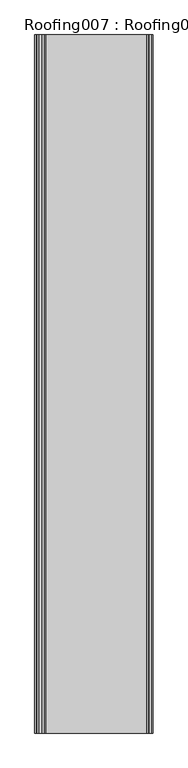
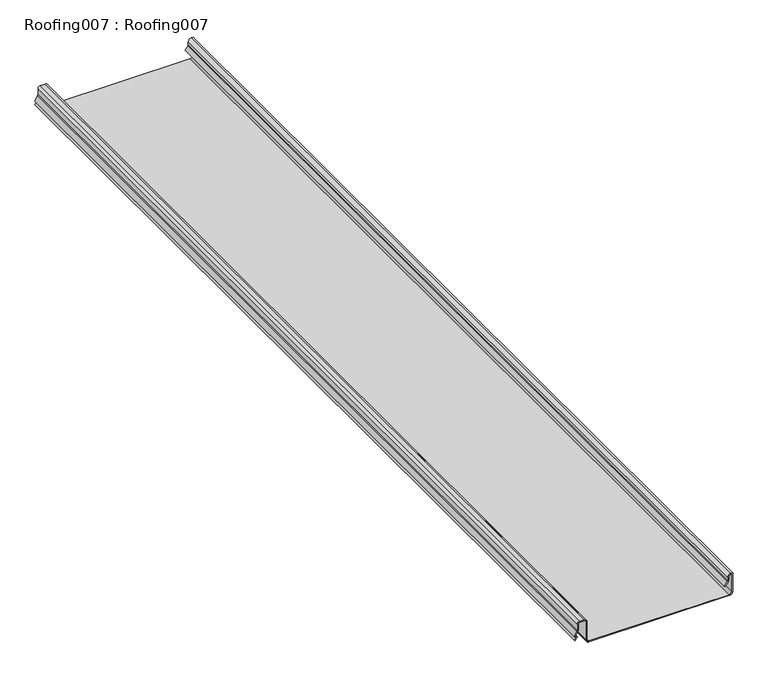
"""IFC4 building model written with IfcOpenShell, lengths in millimetres: proxy geometry, Roofing007 : Roofing007."""

import ifcopenshell
import ifcopenshell.guid

model = None  # the IFC model being written
_history = None  # IfcOwnerHistory: only IFC2X3 demands one
_inside = {}  # id of a spatial element -> (the spatial element, [elements in it])
_under = {}  # id of a project, library or spatial element -> (it, [spatial elements below it])
_declared = {}  # id of a project -> (the project, [libraries it declares])
_typed = {}  # id of a type object -> (the type object, [elements of that type])
_made_of = {}  # id of a material, layer set ... -> (it, [elements and type objects made of it])


def new_model(schema):
    """Start an empty IFC model of exactly this schema.

    Asked for "IFC4X3", IfcOpenShell would pick the latest addendum, in which some entities
    have other attributes; the version numbers below select the first issue.
    IFC2X3 requires an IfcOwnerHistory on every rooted entity: one is made here for all.
    """
    global model, _history
    if schema == "IFC4X3":
        model = ifcopenshell.file(schema_version=(4, 3, 0, 0))
    else:
        model = ifcopenshell.file(schema=schema)
    _inside.clear()
    _under.clear()
    _declared.clear()
    _typed.clear()
    _made_of.clear()
    _history = None
    if model.schema == "IFC2X3":
        org = make("IfcOrganization", Name="unknown")
        user = make(
            "IfcPersonAndOrganization",
            ThePerson=make("IfcPerson", FamilyName="unknown"),
            TheOrganization=org,
        )
        app = make(
            "IfcApplication",
            ApplicationDeveloper=org,
            Version="unknown",
            ApplicationFullName="unknown",
            ApplicationIdentifier="unknown",
        )
        _history = make(
            "IfcOwnerHistory",
            OwningUser=user,
            OwningApplication=app,
            ChangeAction="ADDED",
            CreationDate=0,
        )
    return model


def make(cls, **values):
    """One entity of the class cls with the attributes given. An attribute that is None is left unset."""
    return model.create_entity(
        cls, **{name: value for name, value in values.items() if value is not None}
    )


def rooted(cls, **values):
    """An entity with a GlobalId (a new one), such as an element, a storey or a relation."""
    return make(cls, GlobalId=ifcopenshell.guid.new(), OwnerHistory=_history, **values)


def si_unit(unit_type, name, prefix=None):
    """IfcSIUnit, for example si_unit("LENGTHUNIT", "METRE", prefix="MILLI")."""
    return make("IfcSIUnit", UnitType=unit_type, Prefix=prefix, Name=name)


def assignment(units):
    """IfcUnitAssignment: the units of a project."""
    return None if units is None else make("IfcUnitAssignment", Units=units)


def point(xyz):
    """IfcCartesianPoint."""
    return None if xyz is None else make("IfcCartesianPoint", Coordinates=xyz)


def direction(xyz):
    """IfcDirection."""
    return None if xyz is None else make("IfcDirection", DirectionRatios=xyz)


def frame(location, z_axis=None, x_axis=None):
    """IfcAxis2Placement3D, a coordinate frame: its origin and axes. An axis left out is left unset."""
    return make(
        "IfcAxis2Placement3D",
        Location=point(location),
        Axis=direction(z_axis),
        RefDirection=direction(x_axis),
    )


def frame_2d(location, x_axis=None):
    """IfcAxis2Placement2D, a coordinate frame in the plane: its origin and x axis."""
    return make(
        "IfcAxis2Placement2D", Location=point(location), RefDirection=direction(x_axis)
    )


def origin():
    """The frame at (0, 0, 0) with its axes left unset."""
    return frame((0.0, 0.0, 0.0))


def place(relative_to, where):
    """IfcLocalPlacement: puts the frame where relative to a parent placement (None: the world)."""
    return make(
        "IfcLocalPlacement", PlacementRelTo=relative_to, RelativePlacement=where
    )


def context(
    kind, dimensions, precision=None, world=None, true_north=None, identifier=None
):
    """IfcGeometricRepresentationContext, for example the 3D "Model" context."""
    return make(
        "IfcGeometricRepresentationContext",
        ContextIdentifier=identifier,
        ContextType=kind,
        CoordinateSpaceDimension=dimensions,
        Precision=precision,
        WorldCoordinateSystem=world,
        TrueNorth=true_north,
    )


def project(units=None, contexts=None):
    """IfcProject with its units and contexts."""
    return rooted(
        "IfcProject",
        Name="project",
        RepresentationContexts=contexts,
        UnitsInContext=assignment(units),
    )


def spatial(cls, under=None, at=None, **own):
    """A site, building, storey or space (cls), placed at a placement, below another one or the project."""
    s = rooted(cls, ObjectPlacement=at, **own)
    if under is not None:
        _under.setdefault(under.id(), (under, []))[1].append(s)
    return s


def polyline(points):
    """IfcPolyline through the points."""
    return make("IfcPolyline", Points=[point(p) for p in points])


def circle_curve(where, radius):
    """IfcCircle in the frame where."""
    return make("IfcCircle", Position=where, Radius=radius)


def trimmed(basis, trim1, trim2, sense, master):
    """IfcTrimmedCurve: the piece of a basis curve between two trims."""
    return make(
        "IfcTrimmedCurve",
        BasisCurve=basis,
        Trim1=trim1,
        Trim2=trim2,
        SenseAgreement=sense,
        MasterRepresentation=master,
    )


def segment(curve, same_sense, transition):
    """IfcCompositeCurveSegment."""
    return make(
        "IfcCompositeCurveSegment",
        Transition=transition,
        SameSense=same_sense,
        ParentCurve=curve,
    )


def composite_curve(segments, self_intersect=None):
    """IfcCompositeCurve: segments joined end to end."""
    return make("IfcCompositeCurve", Segments=segments, SelfIntersect=self_intersect)


def outline(outer, holes=None, kind="AREA"):
    """IfcArbitraryClosedProfileDef: a profile drawn as a closed curve; with holes, ...WithVoids."""
    if holes is None:
        return make("IfcArbitraryClosedProfileDef", ProfileType=kind, OuterCurve=outer)
    return make(
        "IfcArbitraryProfileDefWithVoids",
        ProfileType=kind,
        OuterCurve=outer,
        InnerCurves=holes,
    )


def extrude(swept, where, along, depth):
    """IfcExtrudedAreaSolid: the profile swept, set in the frame where, extruded along a direction by depth."""
    return make(
        "IfcExtrudedAreaSolid",
        SweptArea=swept,
        Position=where,
        ExtrudedDirection=direction(along),
        Depth=depth,
    )


def shape(context_of_items, identifier, shape_type, items):
    """IfcShapeRepresentation: the items that make up one representation, for example the "Body"."""
    return make(
        "IfcShapeRepresentation",
        ContextOfItems=context_of_items,
        RepresentationIdentifier=identifier,
        RepresentationType=shape_type,
        Items=items,
    )


def source(mapping_origin, context_of_items, identifier, shape_type, items):
    """IfcRepresentationMap: a shape defined once, which mapped items show again and again."""
    return make(
        "IfcRepresentationMap",
        MappingOrigin=mapping_origin,
        MappedRepresentation=shape(context_of_items, identifier, shape_type, items),
    )


def transform(
    local_origin,
    x_axis=None,
    y_axis=None,
    z_axis=None,
    scale=None,
    scale2=None,
    scale3=None,
    uniform=True,
):
    """IfcCartesianTransformationOperator3D, or its non-uniform kind. x_axis, y_axis, z_axis: its Axis1, 2, 3."""
    if uniform:
        return make(
            "IfcCartesianTransformationOperator3D",
            Axis1=direction(x_axis),
            Axis2=direction(y_axis),
            LocalOrigin=point(local_origin),
            Scale=scale,
            Axis3=direction(z_axis),
        )
    return make(
        "IfcCartesianTransformationOperator3DnonUniform",
        Axis1=direction(x_axis),
        Axis2=direction(y_axis),
        LocalOrigin=point(local_origin),
        Scale=scale,
        Axis3=direction(z_axis),
        Scale2=scale2,
        Scale3=scale3,
    )


def mapped(mapping_source, mapping_target):
    """IfcMappedItem: shows the shape of a source again, moved by a transform."""
    return make(
        "IfcMappedItem", MappingSource=mapping_source, MappingTarget=mapping_target
    )


def made_of(thing, what):
    """Note that an element or type object is made of a material, layer set ...; save() writes the relation."""
    if what is not None:
        _made_of.setdefault(what.id(), (what, []))[1].append(thing)
    return thing


def element(
    cls,
    number,
    at=None,
    inside=None,
    cuts=None,
    type_object=None,
    material=None,
    context=None,
    identifier="Body",
    shape_type=None,
    held_by="IfcProductDefinitionShape",
    body=None,
    shapes=None,
    **own,
):
    """One element of the class cls, such as IfcWall. Its Tag is "e" and its number.

    at: its placement. inside: the storey or other place that contains it. cuts: it is an
    opening in that element (IfcRelVoidsElement). A single representation is given by context,
    identifier, shape_type and body (its items); several are given by shapes. held_by: the class
    of the entity that holds the representations. save() writes the other relations.
    """
    e = rooted(cls, Tag="e%d" % number, ObjectPlacement=at, **own)
    if body is not None:
        shapes = [shape(context, identifier, shape_type, body)]
    if shapes is not None:
        e.Representation = make(held_by, Representations=shapes)
    if inside is not None:
        _inside.setdefault(inside.id(), (inside, []))[1].append(e)
    if cuts is not None:
        rooted(
            "IfcRelVoidsElement", RelatingBuildingElement=cuts, RelatedOpeningElement=e
        )
    if type_object is not None:
        _typed.setdefault(type_object.id(), (type_object, []))[1].append(e)
    return made_of(e, material)


def aggregate(whole, parts):
    """IfcRelAggregates: a whole, such as a stair, and the parts it consists of."""
    return rooted("IfcRelAggregates", RelatingObject=whole, RelatedObjects=parts)


def save(model, path):
    """Write the relations noted so far, then the file.

    IfcRelAggregates (storeys below a building ...), IfcRelContainedInSpatialStructure (elements
    in a storey), IfcRelDefinesByType, IfcRelAssociatesMaterial and IfcRelDeclares: one each for
    every whole, place, type object, material and project.
    """
    for whole, parts in _under.values():
        aggregate(whole, parts)
    for where, things in _inside.values():
        rooted(
            "IfcRelContainedInSpatialStructure",
            RelatedElements=things,
            RelatingStructure=where,
        )
    for kind, things in _typed.values():
        rooted("IfcRelDefinesByType", RelatedObjects=things, RelatingType=kind)
    for what, things in _made_of.values():
        rooted("IfcRelAssociatesMaterial", RelatedObjects=things, RelatingMaterial=what)
    for by, libraries in _declared.values():
        rooted("IfcRelDeclares", RelatingContext=by, RelatedDefinitions=libraries)
    model.write(path)


def roofing007_roofing007_e383adbc(model_context):
    return source(origin(), model_context, "Body", "SweptSolid", [
        extrude(outline(composite_curve([segment(trimmed(circle_curve(frame_2d((42571.8416239, -858.0818689)), 5.08), [point((42568.8585944, -853.969943))], [point((42571.8416239, -853.0018689))], False, "CARTESIAN"), True, "CONTINUOUS"), segment(polyline([(42571.8416239, -853.0018689), (42578.5981823, -853.0018689)]), True, "CONTINUOUS"), segment(trimmed(circle_curve(frame_2d((42578.5981823, -847.9218689)), 5.08), [point((42578.5981823, -853.0018689))], [point((42583.6781823, -847.9218689))], True, "CARTESIAN"), True, "CONTINUOUS"), segment(polyline([(42583.6781823, -847.9218689), (42583.6781823, -846.3270642), (42543.9409948, -846.3270642)]), True, "CONTINUOUS"), segment(trimmed(circle_curve(frame_2d((42543.9409948, -851.4070642)), 5.08), [point((42543.9409948, -846.3270642))], [point((42538.8609948, -851.4070642))], True, "CARTESIAN"), True, "CONTINUOUS"), segment(polyline([(42538.8609948, -851.4070642), (42538.8609948, -1151.6811463)]), True, "CONTINUOUS"), segment(trimmed(circle_curve(frame_2d((42543.9409948, -1151.6811463)), 5.08), [point((42538.8609948, -1151.6811463))], [point((42543.9409948, -1156.7611463))], True, "CARTESIAN"), True, "CONTINUOUS"), segment(polyline([(42543.9409948, -1156.7611463), (42585.5544323, -1156.7611463)]), True, "CONTINUOUS"), segment(trimmed(circle_curve(frame_2d((42585.5544323, -1161.8411463)), 5.08), [point((42585.5544323, -1156.7611463))], [point((42590.6344323, -1161.8411463))], False, "CARTESIAN"), True, "CONTINUOUS"), segment(polyline([(42590.6344323, -1161.8411463), (42590.6344323, -1171.8489232)]), True, "CONTINUOUS"), segment(trimmed(circle_curve(frame_2d((42585.5544323, -1171.8489232)), 5.08), [point((42590.6344323, -1171.8489232))], [point((42585.5544323, -1176.9289232))], False, "CARTESIAN"), True, "CONTINUOUS"), segment(polyline([(42585.5544323, -1176.9289232), (42572.3718581, -1176.9289232)]), True, "CONTINUOUS"), segment(trimmed(circle_curve(frame_2d((42572.3718581, -1182.0089232)), 5.08), [point((42572.3718581, -1176.9289232))], [point((42569.8678467, -1177.5889315))], True, "CARTESIAN"), True, "CONTINUOUS"), segment(polyline([(42569.8678467, -1177.5889315), (42559.3102135, -1183.5700364), (42556.8688073, -1179.4059739), (42551.2672448, -1183.4049974), (42550.1051711, -1181.7772429), (42557.4874863, -1176.5069185), (42560.0388845, -1180.8585833), (42568.8820154, -1175.8487773)]), True, "CONTINUOUS"), segment(trimmed(circle_curve(frame_2d((42572.3718581, -1182.0089232)), 7.08), [point((42568.8820154, -1175.8487773))], [point((42572.3718581, -1174.9289232))], False, "CARTESIAN"), True, "CONTINUOUS"), segment(polyline([(42572.3718581, -1174.9289232), (42585.5544323, -1174.9289232)]), True, "CONTINUOUS"), segment(trimmed(circle_curve(frame_2d((42585.5544323, -1171.8489232)), 3.08), [point((42585.5544323, -1174.9289232))], [point((42588.6344323, -1171.8489232))], True, "CARTESIAN"), True, "CONTINUOUS"), segment(polyline([(42588.6344323, -1171.8489232), (42588.6344323, -1161.8411463)]), True, "CONTINUOUS"), segment(trimmed(circle_curve(frame_2d((42585.5544323, -1161.8411463)), 3.08), [point((42588.6344323, -1161.8411463))], [point((42585.5544323, -1158.7611463))], True, "CARTESIAN"), True, "CONTINUOUS"), segment(polyline([(42585.5544323, -1158.7611463), (42543.9409948, -1158.7611463)]), True, "CONTINUOUS"), segment(trimmed(circle_curve(frame_2d((42543.9409948, -1151.6811463)), 7.08), [point((42543.9409948, -1158.7611463))], [point((42536.8609948, -1151.6811463))], False, "CARTESIAN"), True, "CONTINUOUS"), segment(polyline([(42536.8609948, -1151.6811463), (42536.8609948, -851.4070642)]), True, "CONTINUOUS"), segment(trimmed(circle_curve(frame_2d((42543.9409948, -851.4070642)), 7.08), [point((42536.8609948, -851.4070642))], [point((42543.9409948, -844.3270642))], False, "CARTESIAN"), True, "CONTINUOUS"), segment(polyline([(42543.9409948, -844.3270642), (42585.6781823, -844.3270642), (42585.6781823, -847.9218689)]), True, "CONTINUOUS"), segment(trimmed(circle_curve(frame_2d((42578.5981823, -847.9218689)), 7.08), [point((42585.6781823, -847.9218689))], [point((42578.5981823, -855.0018689))], False, "CARTESIAN"), True, "CONTINUOUS"), segment(polyline([(42578.5981823, -855.0018689), (42571.8416239, -855.0018689)]), True, "CONTINUOUS"), segment(trimmed(circle_curve(frame_2d((42571.8416239, -858.0818689)), 3.08), [point((42571.8416239, -855.0018689))], [point((42570.0330155, -855.5888115))], True, "CARTESIAN"), True, "CONTINUOUS"), segment(polyline([(42570.0330155, -855.5888115), (42561.5588533, -861.7364601), (42560.3844323, -860.1175916), (42568.8585944, -853.969943)]), True, "CONTINUOUS")], self_intersect=False)), frame((0.0, -1052.8906574, 0.0), z_axis=(0.0, 1.0, 0.0), x_axis=(0.0, 0.0, 1.0)), (0.0, 0.0, 1.0), 2000.0),
    ])


if __name__ == "__main__":
    model = new_model("IFC4")
    model_context = context("Model", 3, world=origin())
    ifc_project = project(units=[si_unit("LENGTHUNIT", "METRE", prefix="MILLI")], contexts=[model_context])
    site = spatial("IfcSite", under=ifc_project)
    building = spatial("IfcBuilding", under=site)
    placement = place(None, origin())
    roofing007_roofing007_shape = roofing007_roofing007_e383adbc(model_context)
    element("IfcBuildingElementProxy", 1, Name="Roofing007 : Roofing007", ObjectType="Roofing007 : Roofing007", at=placement, inside=building, context=model_context, shape_type="MappedRepresentation", body=[
        mapped(roofing007_roofing007_shape, transform((0.0, 0.0, 0.0), x_axis=(1.0, 0.0, 0.0), y_axis=(0.0, 1.0, 0.0), z_axis=(0.0, 0.0, 1.0))),
    ])
    save(model, "model.ifc")

# Revit data of these elements
# Type "Roofing007 : Roofing007"
#   NameOverride = "Roofing007"
# Element 1 (IfcBuildingElementProxy, "Roofing007 : Roofing007")
#   Materials on its faces: "STANDING SEAM METAL ROOF FOLLOW MANU. RECOMMENDED EDGE/TRANSITION DETAILS"
# Materials
#   "STANDING SEAM METAL ROOF FOLLOW MANU. RECOMMENDED EDGE/TRANSITION DETAILS": class "Unassigned", colour RGB 128 128 128, transparency 0, Cost = 0
